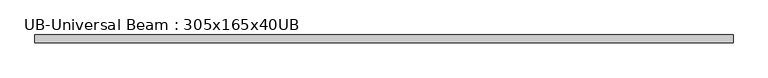
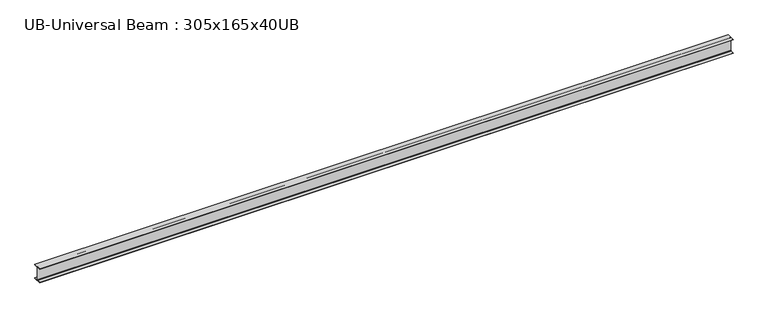
"""IFC4 building model written with IfcOpenShell, lengths in millimetres: beam geometry, UB-Universal Beam : 305x165x40UB."""

from ifc_helpers import new_model, si_unit, point, frame, frame_2d, origin, place, context, project, spatial, polyline, circle_curve, trimmed, segment, composite_curve, outline, extrude, source, transform, mapped, element, save


def ub_universal_beam_305x165x40ub_f67fc52f(model_context):
    return source(origin(), model_context, "Body", "SweptSolid", [
        extrude(outline(composite_curve([segment(polyline([(82.5, -141.5), (82.5, -151.7), (-82.5, -151.7), (-82.5, -141.5), (-11.9, -141.5)]), True, "CONTINUOUS"), segment(trimmed(circle_curve(frame_2d((-11.9, -132.6)), 8.9), [point((-11.9, -141.5))], [point((-3.0, -132.6))], True, "CARTESIAN"), True, "CONTINUOUS"), segment(polyline([(-3.0, -132.6), (-3.0, 132.6)]), True, "CONTINUOUS"), segment(trimmed(circle_curve(frame_2d((-11.9, 132.6)), 8.9), [point((-3.0, 132.6))], [point((-11.9, 141.5))], True, "CARTESIAN"), True, "CONTINUOUS"), segment(polyline([(-11.9, 141.5), (-82.5, 141.5), (-82.5, 151.7), (82.5, 151.7), (82.5, 141.5), (11.9, 141.5)]), True, "CONTINUOUS"), segment(trimmed(circle_curve(frame_2d((11.9, 132.6)), 8.9), [point((11.9, 141.5))], [point((3.0, 132.6))], True, "CARTESIAN"), True, "CONTINUOUS"), segment(polyline([(3.0, 132.6), (3.0, -132.6)]), True, "CONTINUOUS"), segment(trimmed(circle_curve(frame_2d((11.9, -132.6)), 8.9), [point((3.0, -132.6))], [point((11.9, -141.5))], True, "CARTESIAN"), True, "CONTINUOUS"), segment(polyline([(11.9, -141.5), (82.5, -141.5)]), True, "CONTINUOUS")], self_intersect=False)), frame((-7125.0, 0.0, 0.0), z_axis=(1.0, 0.0, 0.0), x_axis=(0.0, 1.0, 0.0)), (0.0, 0.0, 1.0), 14250.0),
    ])


if __name__ == "__main__":
    model = new_model("IFC4")
    model_context = context("Model", 3, world=origin())
    ifc_project = project(units=[si_unit("LENGTHUNIT", "METRE", prefix="MILLI")], contexts=[model_context])
    site = spatial("IfcSite", under=ifc_project)
    building = spatial("IfcBuilding", under=site)
    placement = place(None, origin())
    ub_universal_beam_305x165x40ub_shape = ub_universal_beam_305x165x40ub_f67fc52f(model_context)
    element("IfcBeam", 1, ObjectType="UB-Universal Beam : 305x165x40UB", at=placement, inside=building, context=model_context, shape_type="MappedRepresentation", body=[
        mapped(ub_universal_beam_305x165x40ub_shape, transform((0.0, 0.0, 0.0), x_axis=(1.0, 0.0, 0.0), y_axis=(0.0, 1.0, 0.0), z_axis=(0.0, 0.0, 1.0))),
    ])
    save(model, "model.ifc")

# Revit data of these elements
# Type "UB-Universal Beam : 305x165x40UB"
#   Nominal h = "305"
#   W = 0
#   Start Extension Calculation [instance default] = 3000 mm
#   Start Extension [instance default] = -12.7 mm
#   End Extension Calculation [instance default] = 3000 mm
#   End Extension [instance default] = -12.7 mm
#   Ix = 8503
#   Length [instance default] = 1524 mm
#   M = 40.3
#   Zx = 560
#   b = 165 mm
#   h = 303.4 mm
#   r = 8.9 mm
#   s = 6 mm
#   t = 10.2 mm
#   A = 0.005 m²
#   Structural Material [instance default] = Metal - Steel - 345 MPa
#   Assembly Code = ""
# Element 1 (IfcBeam, "UB-Universal Beam : 305x165x40UB")
#   Materials on its faces: "Metal - Steel - 345 MPa"
# Materials
#   "Metal - Steel - 345 MPa": class "Metal", colour RGB 241 46 46, transparency 0
